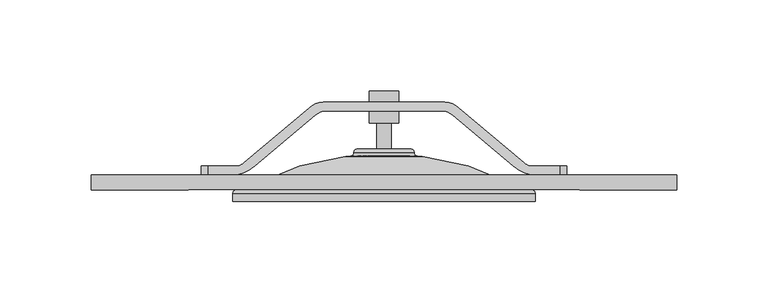
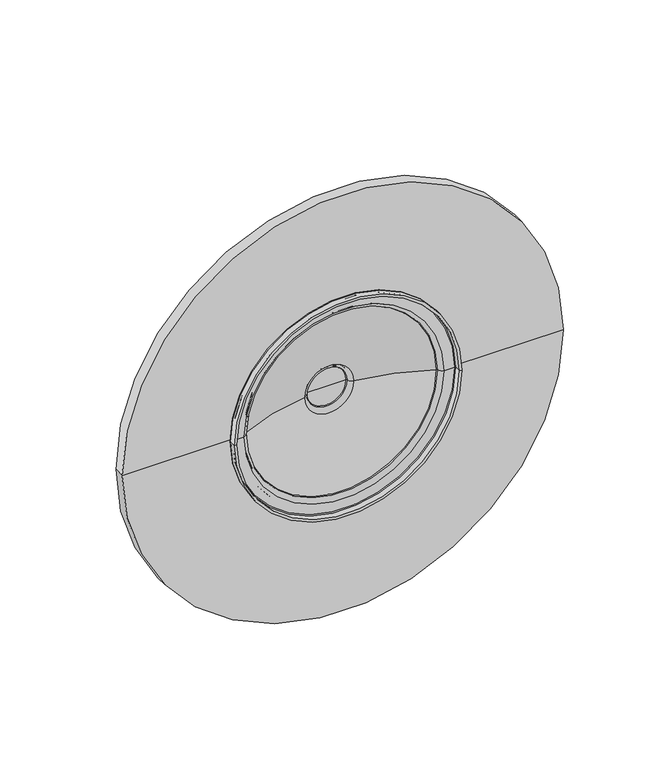
"""IFC4 building model written with IfcOpenShell, lengths in millimetres: proxy geometry, BVNC 300 8Y. : BVNC 300 8Y."""

import ifcopenshell
import ifcopenshell.guid

model = None  # the IFC model being written
_history = None  # IfcOwnerHistory: only IFC2X3 demands one
_inside = {}  # id of a spatial element -> (the spatial element, [elements in it])
_under = {}  # id of a project, library or spatial element -> (it, [spatial elements below it])
_declared = {}  # id of a project -> (the project, [libraries it declares])
_typed = {}  # id of a type object -> (the type object, [elements of that type])
_made_of = {}  # id of a material, layer set ... -> (it, [elements and type objects made of it])


def new_model(schema):
    """Start an empty IFC model of exactly this schema.

    Asked for "IFC4X3", IfcOpenShell would pick the latest addendum, in which some entities
    have other attributes; the version numbers below select the first issue.
    IFC2X3 requires an IfcOwnerHistory on every rooted entity: one is made here for all.
    """
    global model, _history
    if schema == "IFC4X3":
        model = ifcopenshell.file(schema_version=(4, 3, 0, 0))
    else:
        model = ifcopenshell.file(schema=schema)
    _inside.clear()
    _under.clear()
    _declared.clear()
    _typed.clear()
    _made_of.clear()
    _history = None
    if model.schema == "IFC2X3":
        org = make("IfcOrganization", Name="unknown")
        user = make(
            "IfcPersonAndOrganization",
            ThePerson=make("IfcPerson", FamilyName="unknown"),
            TheOrganization=org,
        )
        app = make(
            "IfcApplication",
            ApplicationDeveloper=org,
            Version="unknown",
            ApplicationFullName="unknown",
            ApplicationIdentifier="unknown",
        )
        _history = make(
            "IfcOwnerHistory",
            OwningUser=user,
            OwningApplication=app,
            ChangeAction="ADDED",
            CreationDate=0,
        )
    return model


def make(cls, **values):
    """One entity of the class cls with the attributes given. An attribute that is None is left unset."""
    return model.create_entity(
        cls, **{name: value for name, value in values.items() if value is not None}
    )


def rooted(cls, **values):
    """An entity with a GlobalId (a new one), such as an element, a storey or a relation."""
    return make(cls, GlobalId=ifcopenshell.guid.new(), OwnerHistory=_history, **values)


def si_unit(unit_type, name, prefix=None):
    """IfcSIUnit, for example si_unit("LENGTHUNIT", "METRE", prefix="MILLI")."""
    return make("IfcSIUnit", UnitType=unit_type, Prefix=prefix, Name=name)


def assignment(units):
    """IfcUnitAssignment: the units of a project."""
    return None if units is None else make("IfcUnitAssignment", Units=units)


def point(xyz):
    """IfcCartesianPoint."""
    return None if xyz is None else make("IfcCartesianPoint", Coordinates=xyz)


def direction(xyz):
    """IfcDirection."""
    return None if xyz is None else make("IfcDirection", DirectionRatios=xyz)


def frame(location, z_axis=None, x_axis=None):
    """IfcAxis2Placement3D, a coordinate frame: its origin and axes. An axis left out is left unset."""
    return make(
        "IfcAxis2Placement3D",
        Location=point(location),
        Axis=direction(z_axis),
        RefDirection=direction(x_axis),
    )


def origin():
    """The frame at (0, 0, 0) with its axes left unset."""
    return frame((0.0, 0.0, 0.0))


def place(relative_to, where):
    """IfcLocalPlacement: puts the frame where relative to a parent placement (None: the world)."""
    return make(
        "IfcLocalPlacement", PlacementRelTo=relative_to, RelativePlacement=where
    )


def context(
    kind, dimensions, precision=None, world=None, true_north=None, identifier=None
):
    """IfcGeometricRepresentationContext, for example the 3D "Model" context."""
    return make(
        "IfcGeometricRepresentationContext",
        ContextIdentifier=identifier,
        ContextType=kind,
        CoordinateSpaceDimension=dimensions,
        Precision=precision,
        WorldCoordinateSystem=world,
        TrueNorth=true_north,
    )


def project(units=None, contexts=None):
    """IfcProject with its units and contexts."""
    return rooted(
        "IfcProject",
        Name="project",
        RepresentationContexts=contexts,
        UnitsInContext=assignment(units),
    )


def spatial(cls, under=None, at=None, **own):
    """A site, building, storey or space (cls), placed at a placement, below another one or the project."""
    s = rooted(cls, ObjectPlacement=at, **own)
    if under is not None:
        _under.setdefault(under.id(), (under, []))[1].append(s)
    return s


def polyline(points):
    """IfcPolyline through the points."""
    return make("IfcPolyline", Points=[point(p) for p in points])


def circle_curve(where, radius):
    """IfcCircle in the frame where."""
    return make("IfcCircle", Position=where, Radius=radius)


def ellipse_curve(where, semi_axis1, semi_axis2):
    """IfcEllipse in the frame where."""
    return make(
        "IfcEllipse", Position=where, SemiAxis1=semi_axis1, SemiAxis2=semi_axis2
    )


def trimmed(basis, trim1, trim2, sense, master):
    """IfcTrimmedCurve: the piece of a basis curve between two trims."""
    return make(
        "IfcTrimmedCurve",
        BasisCurve=basis,
        Trim1=trim1,
        Trim2=trim2,
        SenseAgreement=sense,
        MasterRepresentation=master,
    )


def shape(context_of_items, identifier, shape_type, items):
    """IfcShapeRepresentation: the items that make up one representation, for example the "Body"."""
    return make(
        "IfcShapeRepresentation",
        ContextOfItems=context_of_items,
        RepresentationIdentifier=identifier,
        RepresentationType=shape_type,
        Items=items,
    )


def source(mapping_origin, context_of_items, identifier, shape_type, items):
    """IfcRepresentationMap: a shape defined once, which mapped items show again and again."""
    return make(
        "IfcRepresentationMap",
        MappingOrigin=mapping_origin,
        MappedRepresentation=shape(context_of_items, identifier, shape_type, items),
    )


def transform(
    local_origin,
    x_axis=None,
    y_axis=None,
    z_axis=None,
    scale=None,
    scale2=None,
    scale3=None,
    uniform=True,
):
    """IfcCartesianTransformationOperator3D, or its non-uniform kind. x_axis, y_axis, z_axis: its Axis1, 2, 3."""
    if uniform:
        return make(
            "IfcCartesianTransformationOperator3D",
            Axis1=direction(x_axis),
            Axis2=direction(y_axis),
            LocalOrigin=point(local_origin),
            Scale=scale,
            Axis3=direction(z_axis),
        )
    return make(
        "IfcCartesianTransformationOperator3DnonUniform",
        Axis1=direction(x_axis),
        Axis2=direction(y_axis),
        LocalOrigin=point(local_origin),
        Scale=scale,
        Axis3=direction(z_axis),
        Scale2=scale2,
        Scale3=scale3,
    )


def mapped(mapping_source, mapping_target):
    """IfcMappedItem: shows the shape of a source again, moved by a transform."""
    return make(
        "IfcMappedItem", MappingSource=mapping_source, MappingTarget=mapping_target
    )


def made_of(thing, what):
    """Note that an element or type object is made of a material, layer set ...; save() writes the relation."""
    if what is not None:
        _made_of.setdefault(what.id(), (what, []))[1].append(thing)
    return thing


def element(
    cls,
    number,
    at=None,
    inside=None,
    cuts=None,
    type_object=None,
    material=None,
    context=None,
    identifier="Body",
    shape_type=None,
    held_by="IfcProductDefinitionShape",
    body=None,
    shapes=None,
    **own,
):
    """One element of the class cls, such as IfcWall. Its Tag is "e" and its number.

    at: its placement. inside: the storey or other place that contains it. cuts: it is an
    opening in that element (IfcRelVoidsElement). A single representation is given by context,
    identifier, shape_type and body (its items); several are given by shapes. held_by: the class
    of the entity that holds the representations. save() writes the other relations.
    """
    e = rooted(cls, Tag="e%d" % number, ObjectPlacement=at, **own)
    if body is not None:
        shapes = [shape(context, identifier, shape_type, body)]
    if shapes is not None:
        e.Representation = make(held_by, Representations=shapes)
    if inside is not None:
        _inside.setdefault(inside.id(), (inside, []))[1].append(e)
    if cuts is not None:
        rooted(
            "IfcRelVoidsElement", RelatingBuildingElement=cuts, RelatedOpeningElement=e
        )
    if type_object is not None:
        _typed.setdefault(type_object.id(), (type_object, []))[1].append(e)
    return made_of(e, material)


def aggregate(whole, parts):
    """IfcRelAggregates: a whole, such as a stair, and the parts it consists of."""
    return rooted("IfcRelAggregates", RelatingObject=whole, RelatedObjects=parts)


def save(model, path):
    """Write the relations noted so far, then the file.

    IfcRelAggregates (storeys below a building ...), IfcRelContainedInSpatialStructure (elements
    in a storey), IfcRelDefinesByType, IfcRelAssociatesMaterial and IfcRelDeclares: one each for
    every whole, place, type object, material and project.
    """
    for whole, parts in _under.values():
        aggregate(whole, parts)
    for where, things in _inside.values():
        rooted(
            "IfcRelContainedInSpatialStructure",
            RelatedElements=things,
            RelatingStructure=where,
        )
    for kind, things in _typed.values():
        rooted("IfcRelDefinesByType", RelatedObjects=things, RelatingType=kind)
    for what, things in _made_of.values():
        rooted("IfcRelAssociatesMaterial", RelatedObjects=things, RelatingMaterial=what)
    for by, libraries in _declared.values():
        rooted("IfcRelDeclares", RelatingContext=by, RelatedDefinitions=libraries)
    model.write(path)


def plane_surface(at):
    """IfcPlane: the flat surface through the origin of the frame at, square to its z axis."""
    return make("IfcPlane", Position=at)


def cylinder_surface(at, radius):
    """IfcCylindricalSurface: all points at the distance radius from the z axis of the frame at."""
    return make("IfcCylindricalSurface", Position=at, Radius=radius)


def revolved_surface(curve, axis_point, axis_direction):
    """IfcSurfaceOfRevolution: the curve turned about the line through axis_point along axis_direction."""
    return make(
        "IfcSurfaceOfRevolution",
        SweptCurve=make("IfcArbitraryOpenProfileDef", ProfileType="CURVE", Curve=curve),
        AxisPosition=make("IfcAxis1Placement", Location=point(axis_point), Axis=direction(axis_direction)),
    )


def advanced_brep(points, edges, surfaces, faces):
    """IfcAdvancedBrep: a solid bounded by faces that lie on surfaces and meet in shared edges.

    An edge is (start, end): straight between two places in points (the first is 0);
    or (start, end, curve); or (start, end, curve, False) where it runs against its curve.
    A face is (place in surfaces, loops), or (place, loops, False) where it looks against
    its surface's normal. A loop lists edges by number (the first is 1), with a minus sign
    where the edge is run from its end to its start. The first loop is the outer one.
    """
    corners = [point(p) for p in points]
    vertices = [make("IfcVertexPoint", VertexGeometry=c) for c in corners]
    made = []
    for start, end, *more in edges:
        made.append(
            make(
                "IfcEdgeCurve",
                EdgeStart=vertices[start],
                EdgeEnd=vertices[end],
                EdgeGeometry=more[0] if more else make("IfcPolyline", Points=[corners[start], corners[end]]),
                SameSense=more[1] if len(more) > 1 else True,
            )
        )
    hull = []
    for where, loops, *sense in faces:
        bounds = []
        for j, loop in enumerate(loops):
            ring = [make("IfcOrientedEdge", EdgeElement=made[abs(k) - 1], Orientation=k > 0) for k in loop]
            bounds.append(
                make(
                    "IfcFaceOuterBound" if j == 0 else "IfcFaceBound",
                    Bound=make("IfcEdgeLoop", EdgeList=ring),
                    Orientation=True,
                )
            )
        hull.append(make("IfcAdvancedFace", Bounds=bounds, FaceSurface=surfaces[where], SameSense=sense[0] if sense else True))
    return make("IfcAdvancedBrep", Outer=make("IfcClosedShell", CfsFaces=hull))


def mechanical_equipment_0198ac86(model_context):
    return source(origin(), model_context, "Body", "AdvancedBrep", [
        advanced_brep(
        [(44.3795006, 108.0, 2510.0), (54.2298211, 113.0, 2510.0), (87.44309, 140.8692417, 2510.0), (91.8102497, 143.0, 2510.0), (125.0, 143.0, 2510.0), (158.1897503, 143.0, 2510.0), (162.55691, 140.8692417, 2510.0), (195.7701789, 113.0, 2510.0), (205.6204994, 108.0, 2510.0), (221.2200072, 108.0, 2510.0), (221.2200072, 113.0, 2510.0), (205.6204994, 113.0, 2510.0), (201.5540671, 114.8851429, 2510.0), (165.874925, 144.8234979, 2510.0), (158.1897503, 148.0, 2510.0), (125.0, 148.0, 2510.0), (91.8102497, 148.0, 2510.0), (84.125075, 144.8234979, 2510.0), (48.4459329, 114.8851429, 2510.0), (44.3795006, 113.0, 2510.0), (28.7799928, 113.0, 2510.0), (28.7799928, 108.0, 2510.0), (44.3795006, 113.0, 2490.0), (48.4459329, 114.8851429, 2490.0), (84.125075, 144.8234979, 2490.0), (91.8102497, 148.0, 2490.0), (125.0, 148.0, 2490.0), (158.1897503, 148.0, 2490.0), (165.874925, 144.8234979, 2490.0), (201.5540671, 114.8851429, 2490.0), (205.6204994, 113.0, 2490.0), (221.2200072, 113.0, 2490.0), (221.2200072, 108.0, 2490.0), (205.6204994, 108.0, 2490.0), (195.7701789, 113.0, 2490.0), (162.55691, 140.8692417, 2490.0), (158.1897503, 143.0, 2490.0), (125.0, 143.0, 2490.0), (91.8102497, 143.0, 2490.0), (87.44309, 140.8692417, 2490.0), (54.2298211, 113.0, 2490.0), (44.3795006, 108.0, 2490.0), (28.7799928, 108.0, 2490.0), (28.7799928, 113.0, 2490.0), (25.0, 108.0, 2506.2200072), (25.0, 108.0, 2493.7799928), (225.0, 108.0, 2493.7799928), (225.0, 108.0, 2506.2200072), (225.0, 113.0, 2493.7799928), (225.0, 113.0, 2506.2200072), (25.0, 113.0, 2493.7799928), (25.0, 113.0, 2506.2200072)],
        [
            (0, 1, circle_curve(frame((38.5511411, 131.6851233, 2510.0), z_axis=(0.0, 0.0, 1.0), x_axis=(1.0, 0.0, 0.0)), 24.3916961)),
            (1, 2),
            (2, 3, circle_curve(frame((93.9022065, 133.1715663, 2510.0), z_axis=(0.0, 0.0, -1.0), x_axis=(1.0, 0.0, 0.0)), 10.0486015)),
            (3, 4),
            (4, 5),
            (5, 6, circle_curve(frame((156.0977935, 133.1715663, 2510.0), z_axis=(0.0, 0.0, -1.0), x_axis=(-1.0, 0.0, 0.0)), 10.0486015)),
            (6, 7),
            (7, 8, circle_curve(frame((211.4488589, 131.6851233, 2510.0), z_axis=(0.0, 0.0, 1.0), x_axis=(-1.0, 0.0, 0.0)), 24.3916961)),
            (8, 9),
            (9, 10),
            (10, 11),
            (11, 12, circle_curve(frame((205.6204994, 118.3284116, 2510.0), z_axis=(0.0, 0.0, -1.0), x_axis=(-1.0, 0.0, 0.0)), 5.3284116)),
            (12, 13),
            (13, 14, circle_curve(frame((158.1897503, 137.115059, 2510.0), z_axis=(0.0, 0.0, 1.0), x_axis=(-1.0, 0.0, 0.0)), 10.884941)),
            (14, 15),
            (15, 16),
            (16, 17, circle_curve(frame((91.8102497, 137.115059, 2510.0), z_axis=(0.0, 0.0, 1.0), x_axis=(1.0, 0.0, 0.0)), 10.884941)),
            (17, 18),
            (18, 19, circle_curve(frame((44.3795006, 118.3284116, 2510.0), z_axis=(0.0, 0.0, -1.0), x_axis=(1.0, 0.0, 0.0)), 5.3284116)),
            (19, 20),
            (20, 21),
            (21, 0),
            (22, 23, circle_curve(frame((44.3795006, 118.3284116, 2490.0), z_axis=(0.0, 0.0, 1.0), x_axis=(1.0, 0.0, 0.0)), 5.3284116)),
            (23, 24),
            (24, 25, circle_curve(frame((91.8102497, 137.115059, 2490.0), z_axis=(0.0, 0.0, -1.0), x_axis=(1.0, 0.0, 0.0)), 10.884941)),
            (25, 26),
            (26, 27),
            (27, 28, circle_curve(frame((158.1897503, 137.115059, 2490.0), z_axis=(0.0, 0.0, -1.0), x_axis=(-1.0, 0.0, 0.0)), 10.884941)),
            (28, 29),
            (29, 30, circle_curve(frame((205.6204994, 118.3284116, 2490.0), z_axis=(0.0, 0.0, 1.0), x_axis=(-1.0, 0.0, 0.0)), 5.3284116)),
            (30, 31),
            (31, 32),
            (32, 33),
            (33, 34, circle_curve(frame((211.4488589, 131.6851233, 2490.0), z_axis=(0.0, 0.0, -1.0), x_axis=(-1.0, 0.0, 0.0)), 24.3916961)),
            (34, 35),
            (35, 36, circle_curve(frame((156.0977935, 133.1715663, 2490.0), z_axis=(0.0, 0.0, 1.0), x_axis=(-1.0, 0.0, 0.0)), 10.0486015)),
            (36, 37),
            (37, 38),
            (38, 39, circle_curve(frame((93.9022065, 133.1715663, 2490.0), z_axis=(0.0, 0.0, 1.0), x_axis=(1.0, 0.0, 0.0)), 10.0486015)),
            (39, 40),
            (40, 41, circle_curve(frame((38.5511411, 131.6851233, 2490.0), z_axis=(0.0, 0.0, -1.0), x_axis=(1.0, 0.0, 0.0)), 24.3916961)),
            (41, 42),
            (42, 43),
            (43, 22),
            (41, 0),
            (21, 44, circle_curve(frame((28.7799928, 108.0, 2506.2200072), z_axis=(0.0, -1.0, 0.0), x_axis=(1.0, 0.0, 0.0)), 3.7799928)),
            (44, 45),
            (45, 42, circle_curve(frame((28.7799928, 108.0, 2493.7799928), z_axis=(0.0, -1.0, 0.0), x_axis=(1.0, 0.0, 0.0)), 3.7799928)),
            (40, 1),
            (39, 2),
            (38, 3),
            (37, 4),
            (36, 5),
            (35, 6),
            (34, 7),
            (33, 8),
            (32, 46, circle_curve(frame((221.2200072, 108.0, 2493.7799928), z_axis=(0.0, -1.0, 0.0), x_axis=(-1.0, 0.0, 0.0)), 3.7799928)),
            (46, 47),
            (47, 9, circle_curve(frame((221.2200072, 108.0, 2506.2200072), z_axis=(0.0, -1.0, 0.0), x_axis=(-1.0, 0.0, 0.0)), 3.7799928)),
            (46, 48),
            (48, 49),
            (49, 47),
            (30, 11),
            (10, 49, circle_curve(frame((221.2200072, 113.0, 2506.2200072), z_axis=(0.0, 1.0, 0.0), x_axis=(-1.0, 0.0, 0.0)), 3.7799928)),
            (48, 31, circle_curve(frame((221.2200072, 113.0, 2493.7799928), z_axis=(0.0, 1.0, 0.0), x_axis=(-1.0, 0.0, 0.0)), 3.7799928)),
            (29, 12),
            (28, 13),
            (27, 14),
            (26, 15),
            (25, 16),
            (24, 17),
            (23, 18),
            (22, 19),
            (43, 50, circle_curve(frame((28.7799928, 113.0, 2493.7799928), z_axis=(0.0, 1.0, 0.0), x_axis=(1.0, 0.0, 0.0)), 3.7799928)),
            (50, 51),
            (51, 20, circle_curve(frame((28.7799928, 113.0, 2506.2200072), z_axis=(0.0, 1.0, 0.0), x_axis=(1.0, 0.0, 0.0)), 3.7799928)),
            (44, 51),
            (50, 45),
        ],
        [
            plane_surface(frame((25.0, 108.0, 2510.0), z_axis=(0.0, 0.0, 1.0), x_axis=(1.0, 0.0, 0.0))),
            plane_surface(frame((25.0, 108.0, 2490.0), z_axis=(0.0, 0.0, -1.0), x_axis=(-1.0, 0.0, 0.0))),
            plane_surface(frame((25.0, 108.0, 2510.0), z_axis=(0.0, -1.0, 0.0), x_axis=(0.0, 0.0, -1.0))),
            cylinder_surface(frame((38.5511411, 131.6851233, 2490.0), z_axis=(0.0, 0.0, 1.0), x_axis=(1.0, 0.0, 0.0)), 24.3916961),
            plane_surface(frame((54.2298211, 113.0, 2510.0), z_axis=(0.6427876096865391, -0.7660444431189783, 0.0), x_axis=(0.0, 0.0, -1.0))),
            revolved_surface(polyline([(103.95080800000001, 133.1715663, 2490.0), (103.95080800000001, 133.1715663, 2510.0)]), (93.9022065, 133.1715663, 2490.0), (0.0, 0.0, -1.0)),
            plane_surface(frame((91.8102497, 143.0, 2510.0), z_axis=(0.0, -1.0, 0.0), x_axis=(0.0, 0.0, -1.0))),
            plane_surface(frame((125.0, 143.0, 2510.0), z_axis=(0.0, -1.0, 0.0), x_axis=(0.0, 0.0, -1.0))),
            revolved_surface(polyline([(146.049192, 133.1715663, 2490.0), (146.049192, 133.1715663, 2510.0)]), (156.0977935, 133.1715663, 2490.0), (0.0, 0.0, -1.0)),
            plane_surface(frame((162.55691, 140.8692417, 2510.0), z_axis=(-0.6427876096865387, -0.7660444431189786, 0.0), x_axis=(0.0, 0.0, -1.0))),
            cylinder_surface(frame((211.4488589, 131.6851233, 2490.0), z_axis=(0.0, 0.0, 1.0), x_axis=(-1.0, 0.0, 0.0)), 24.3916961),
            plane_surface(frame((205.6204994, 108.0, 2510.0), z_axis=(0.0, -1.0, 0.0), x_axis=(0.0, 0.0, -1.0))),
            plane_surface(frame((225.0, 108.0, 2510.0), z_axis=(1.0, 0.0, 0.0), x_axis=(0.0, 0.0, -1.0))),
            plane_surface(frame((225.0, 113.0, 2510.0), z_axis=(0.0, 1.0, 0.0), x_axis=(0.0, 0.0, -1.0))),
            revolved_surface(polyline([(200.2920878, 118.3284116, 2490.0), (200.2920878, 118.3284116, 2510.0)]), (205.6204994, 118.3284116, 2490.0), (0.0, 0.0, -1.0)),
            plane_surface(frame((201.5540671, 114.8851429, 2510.0), z_axis=(0.6427876096865414, 0.7660444431189763, 0.0), x_axis=(0.0, 0.0, -1.0))),
            cylinder_surface(frame((158.1897503, 137.115059, 2490.0), z_axis=(0.0, 0.0, 1.0), x_axis=(-1.0, 0.0, 0.0)), 10.884941),
            plane_surface(frame((158.1897503, 148.0, 2510.0), z_axis=(0.0, 1.0, 0.0), x_axis=(0.0, 0.0, -1.0))),
            plane_surface(frame((125.0, 148.0, 2510.0), z_axis=(0.0, 1.0, 0.0), x_axis=(0.0, 0.0, -1.0))),
            cylinder_surface(frame((91.8102497, 137.115059, 2490.0), z_axis=(0.0, 0.0, 1.0), x_axis=(1.0, 0.0, 0.0)), 10.884941),
            plane_surface(frame((84.125075, 144.8234979, 2510.0), z_axis=(-0.6427876096865359, 0.766044443118981, 0.0), x_axis=(0.0, 0.0, -1.0))),
            revolved_surface(polyline([(49.7079122, 118.3284116, 2490.0), (49.7079122, 118.3284116, 2510.0)]), (44.3795006, 118.3284116, 2490.0), (0.0, 0.0, -1.0)),
            plane_surface(frame((44.3795006, 113.0, 2510.0), z_axis=(0.0, 1.0, 0.0), x_axis=(0.0, 0.0, -1.0))),
            plane_surface(frame((25.0, 113.0, 2510.0), z_axis=(-1.0, 0.0, 0.0), x_axis=(0.0, 0.0, -1.0))),
            cylinder_surface(frame((28.7799928, 108.0, 2493.7799928), z_axis=(0.0, -1.0, 0.0), x_axis=(1.0, 0.0, 0.0)), 3.7799928),
            cylinder_surface(frame((28.7799928, 93.5, 2506.2200072), z_axis=(0.0, -1.0, 0.0), x_axis=(1.0, 0.0, 0.0)), 3.7799928),
            cylinder_surface(frame((221.2200072, 93.5, 2493.7799928), z_axis=(0.0, -1.0, 0.0), x_axis=(-1.0, 0.0, 0.0)), 3.7799928),
            cylinder_surface(frame((221.2200072, 93.5, 2506.2200072), z_axis=(0.0, -1.0, 0.0), x_axis=(-1.0, 0.0, 0.0)), 3.7799928),
        ],
        [
            (0, [[1, 2, 3, 4, 5, 6, 7, 8, 9, 10, 11, 12, 13, 14, 15, 16, 17, 18, 19, 20, 21, 22]]),
            (1, [[23, 24, 25, 26, 27, 28, 29, 30, 31, 32, 33, 34, 35, 36, 37, 38, 39, 40, 41, 42, 43, 44]]),
            (2, [[45, -22, 46, 47, 48, -42]]),
            (3, [[-1, -45, -41, 49]]),
            (4, [[-2, -49, -40, 50]]),
            (5, [[-3, -50, -39, 51]]),
            (6, [[-4, -51, -38, 52]]),
            (7, [[-5, -52, -37, 53]]),
            (8, [[-6, -53, -36, 54]]),
            (9, [[-7, -54, -35, 55]]),
            (10, [[-8, -55, -34, 56]]),
            (11, [[-56, -33, 57, 58, 59, -9]]),
            (12, [[-58, 60, 61, 62]]),
            (13, [[63, -11, 64, -61, 65, -31]]),
            (14, [[-12, -63, -30, 66]]),
            (15, [[-13, -66, -29, 67]]),
            (16, [[-14, -67, -28, 68]]),
            (17, [[-15, -68, -27, 69]]),
            (18, [[-16, -69, -26, 70]]),
            (19, [[-17, -70, -25, 71]]),
            (20, [[-18, -71, -24, 72]]),
            (21, [[-19, -72, -23, 73]]),
            (22, [[-73, -44, 74, 75, 76, -20]]),
            (23, [[-47, 77, -75, 78]]),
            (24, [[-43, -48, -78, -74]]),
            (25, [[-21, -76, -77, -46]]),
            (26, [[-32, -65, -60, -57]]),
            (27, [[-10, -59, -62, -64]]),
        ],
    ),
        advanced_brep(
        [(207.7271571, 93.5, 2500.0), (42.2728429, 93.5, 2500.0), (42.2728429, 97.7728429, 2500.0), (207.7271571, 97.7728429, 2500.0), (205.9367462, 93.5, 2500.0), (44.0632538, 93.5, 2500.0), (205.9367462, 97.9071057, 2500.0), (44.0632538, 97.9071057, 2500.0), (205.3438519, 98.5, 2500.0), (44.6561481, 98.5, 2500.0), (197.7785514, 98.5, 2500.0), (52.2214486, 98.5, 2500.0), (194.5390342, 101.1233093, 2500.0), (55.4609658, 101.1233093, 2500.0), (194.110594, 101.9290881, 2500.0), (55.889406, 101.9290881, 2500.0), (143.1174907, 117.056758, 2500.0), (106.8825093, 117.056758, 2500.0), (139.9690463, 120.2052024, 2500.0), (110.0309537, 120.2052024, 2500.0), (139.3942487, 120.78, 2500.0), (110.6057513, 120.78, 2500.0), (125.0, 120.78, 2500.0), (139.6388233, 122.2731901, 2500.0), (110.3611767, 122.2731901, 2500.0), (120.9566338, 122.2731901, 2500.0), (129.0433662, 122.2731901, 2500.0), (141.5029828, 120.4090307, 2500.0), (108.4970172, 120.4090307, 2500.0), (143.1991524, 118.522856, 2500.0), (106.8008476, 118.522856, 2500.0), (145.9642188, 118.2410596, 2500.0), (104.0357812, 118.2410596, 2500.0), (194.877574, 103.206216, 2500.0), (55.122426, 103.206216, 2500.0), (196.1038029, 101.6367146, 2500.0), (53.8961971, 101.6367146, 2500.0), (198.0543634, 100.0, 2500.0), (51.9456366, 100.0, 2500.0), (200.0, 100.0, 2500.0), (50.0, 100.0, 2500.0), (200.0, 108.0, 2500.0), (50.0, 108.0, 2500.0), (285.0, 108.0, 2500.0), (-35.0, 108.0, 2500.0), (285.0, 100.0, 2500.0), (-35.0, 100.0, 2500.0), (205.5, 100.0, 2500.0), (44.5, 100.0, 2500.0), (133.0867323, 136.6576943, 2500.0), (116.9132677, 136.6576943, 2500.0), (116.9132677, 153.9, 2500.0), (133.0867323, 153.9, 2500.0), (129.0433662, 136.6576943, 2500.0), (120.9566338, 136.6576943, 2500.0), (125.0, 153.9, 2500.0)],
        [
            (0, 1, circle_curve(frame((125.0, 93.5, 2500.0), z_axis=(0.0, 1.0, 0.0), x_axis=(-1.0, 0.0, 0.0)), 82.7271571)),
            (1, 2),
            (2, 3, circle_curve(frame((125.0, 97.7728429, 2500.0), z_axis=(0.0, -1.0, 0.0), x_axis=(-1.0, 0.0, 0.0)), 82.7271571)),
            (3, 0),
            (1, 0, circle_curve(frame((125.0, 93.5, 2500.0), z_axis=(0.0, 1.0, 0.0), x_axis=(-1.0, 0.0, 0.0)), 82.7271571)),
            (3, 2, circle_curve(frame((125.0, 97.7728429, 2500.0), z_axis=(0.0, -1.0, 0.0), x_axis=(-1.0, 0.0, 0.0)), 82.7271571)),
            (0, 4),
            (4, 5, circle_curve(frame((125.0, 93.5, 2500.0), z_axis=(0.0, 1.0, 0.0), x_axis=(-1.0, 0.0, 0.0)), 80.9367462)),
            (5, 1),
            (5, 4, circle_curve(frame((125.0, 93.5, 2500.0), z_axis=(0.0, 1.0, 0.0), x_axis=(-1.0, 0.0, 0.0)), 80.9367462)),
            (4, 6),
            (6, 7, circle_curve(frame((125.0, 97.9071057, 2500.0), z_axis=(0.0, 1.0, 0.0), x_axis=(-1.0, 0.0, 0.0)), 80.9367462)),
            (7, 5),
            (7, 6, circle_curve(frame((125.0, 97.9071057, 2500.0), z_axis=(0.0, 1.0, 0.0), x_axis=(-1.0, 0.0, 0.0)), 80.9367462)),
            (6, 8, circle_curve(frame((205.3438519, 97.9071057, 2500.0), z_axis=(0.0, 0.0, 1.0), x_axis=(-1.0, 0.0, 0.0)), 0.5928943)),
            (8, 9, circle_curve(frame((125.0, 98.5, 2500.0), z_axis=(0.0, 1.0, 0.0), x_axis=(-1.0, 0.0, 0.0)), 80.3438519)),
            (9, 7, circle_curve(frame((44.6561481, 97.9071057, 2500.0), z_axis=(0.0, 0.0, 1.0), x_axis=(1.0, 0.0, 0.0)), 0.5928943)),
            (9, 8, circle_curve(frame((125.0, 98.5, 2500.0), z_axis=(0.0, 1.0, 0.0), x_axis=(-1.0, 0.0, 0.0)), 80.3438519)),
            (8, 10),
            (10, 11, circle_curve(frame((125.0, 98.5, 2500.0), z_axis=(0.0, 1.0, 0.0), x_axis=(-1.0, 0.0, 0.0)), 72.7785514)),
            (11, 9),
            (11, 10, circle_curve(frame((125.0, 98.5, 2500.0), z_axis=(0.0, 1.0, 0.0), x_axis=(-1.0, 0.0, 0.0)), 72.7785514)),
            (10, 12, circle_curve(frame((197.9467336, 102.0195777, 2500.0), z_axis=(0.0, 0.0, -1.0), x_axis=(-1.0, 0.0, 0.0)), 3.5235937)),
            (12, 13, circle_curve(frame((125.0, 101.1233093, 2500.0), z_axis=(0.0, 1.0, 0.0), x_axis=(-1.0, 0.0, 0.0)), 69.5390342)),
            (13, 11, circle_curve(frame((52.0532664, 102.0195777, 2500.0), z_axis=(0.0, 0.0, -1.0), x_axis=(1.0, 0.0, 0.0)), 3.5235937)),
            (13, 12, circle_curve(frame((125.0, 101.1233093, 2500.0), z_axis=(0.0, 1.0, 0.0), x_axis=(-1.0, 0.0, 0.0)), 69.5390342)),
            (12, 14, circle_curve(frame((193.7458269, 101.2183458, 2500.0), z_axis=(0.0, 0.0, 1.0), x_axis=(-1.0, 0.0, 0.0)), 0.7988803)),
            (14, 15, circle_curve(frame((125.0, 101.9290881, 2500.0), z_axis=(0.0, 1.0, 0.0), x_axis=(-1.0, 0.0, 0.0)), 69.110594)),
            (15, 13, circle_curve(frame((56.2541731, 101.2183458, 2500.0), z_axis=(0.0, 0.0, 1.0), x_axis=(1.0, 0.0, 0.0)), 0.7988803)),
            (15, 14, circle_curve(frame((125.0, 101.9290881, 2500.0), z_axis=(0.0, 1.0, 0.0), x_axis=(-1.0, 0.0, 0.0)), 69.110594)),
            (14, 16, circle_curve(frame((128.3688639, -26.1675298, 2500.0), z_axis=(0.0, 0.0, 1.0), x_axis=(-1.0, 0.0, 0.0)), 143.9816606)),
            (16, 17, circle_curve(frame((125.0, 117.056758, 2500.0), z_axis=(0.0, 1.0, 0.0), x_axis=(-1.0, 0.0, 0.0)), 18.1174907)),
            (17, 15, circle_curve(frame((121.6311361, -26.1675298, 2500.0), z_axis=(0.0, 0.0, 1.0), x_axis=(1.0, 0.0, 0.0)), 143.9816606)),
            (17, 16, circle_curve(frame((125.0, 117.056758, 2500.0), z_axis=(0.0, 1.0, 0.0), x_axis=(-1.0, 0.0, 0.0)), 18.1174907)),
            (16, 18, circle_curve(frame((143.1174907, 120.2052024, 2500.0), z_axis=(0.0, 0.0, -1.0), x_axis=(-1.0, 0.0, 0.0)), 3.1484444)),
            (18, 19, circle_curve(frame((125.0, 120.2052024, 2500.0), z_axis=(0.0, 1.0, 0.0), x_axis=(-1.0, 0.0, 0.0)), 14.9690463)),
            (19, 17, circle_curve(frame((106.8825093, 120.2052024, 2500.0), z_axis=(0.0, 0.0, -1.0), x_axis=(1.0, 0.0, 0.0)), 3.1484444)),
            (19, 18, circle_curve(frame((125.0, 120.2052024, 2500.0), z_axis=(0.0, 1.0, 0.0), x_axis=(-1.0, 0.0, 0.0)), 14.9690463)),
            (18, 20, circle_curve(frame((139.3942487, 120.2052024, 2500.0), z_axis=(0.0, 0.0, 1.0), x_axis=(-1.0, 0.0, 0.0)), 0.5747976)),
            (20, 21, circle_curve(frame((125.0, 120.78, 2500.0), z_axis=(0.0, 1.0, 0.0), x_axis=(-1.0, 0.0, 0.0)), 14.3942487)),
            (21, 19, circle_curve(frame((110.6057513, 120.2052024, 2500.0), z_axis=(0.0, 0.0, 1.0), x_axis=(1.0, 0.0, 0.0)), 0.5747976)),
            (21, 20, circle_curve(frame((125.0, 120.78, 2500.0), z_axis=(0.0, 1.0, 0.0), x_axis=(-1.0, 0.0, 0.0)), 14.3942487)),
            (20, 22),
            (22, 21),
            (23, 24, circle_curve(frame((125.0, 122.2731901, 2500.0), z_axis=(0.0, 1.0, 0.0), x_axis=(-1.0, 0.0, 0.0)), 14.6388233)),
            (24, 25),
            (25, 26, circle_curve(frame((125.0, 122.2731901, 2500.0), z_axis=(0.0, -1.0, 0.0), x_axis=(-1.0, 0.0, 0.0)), 4.0433662)),
            (26, 23),
            (24, 23, circle_curve(frame((125.0, 122.2731901, 2500.0), z_axis=(0.0, 1.0, 0.0), x_axis=(-1.0, 0.0, 0.0)), 14.6388233)),
            (26, 25, circle_curve(frame((125.0, 122.2731901, 2500.0), z_axis=(0.0, -1.0, 0.0), x_axis=(-1.0, 0.0, 0.0)), 4.0433662)),
            (23, 27, circle_curve(frame((139.6388233, 120.4090307, 2500.0), z_axis=(0.0, 0.0, -1.0), x_axis=(-1.0, 0.0, 0.0)), 1.8641595)),
            (27, 28, circle_curve(frame((125.0, 120.4090307, 2500.0), z_axis=(0.0, 1.0, 0.0), x_axis=(-1.0, 0.0, 0.0)), 16.5029828)),
            (28, 24, circle_curve(frame((110.3611767, 120.4090307, 2500.0), z_axis=(0.0, 0.0, -1.0), x_axis=(1.0, 0.0, 0.0)), 1.8641595)),
            (28, 27, circle_curve(frame((125.0, 120.4090307, 2500.0), z_axis=(0.0, 1.0, 0.0), x_axis=(-1.0, 0.0, 0.0)), 16.5029828)),
            (27, 29, circle_curve(frame((143.3997997, 120.4090307, 2500.0), z_axis=(0.0, 0.0, 1.0), x_axis=(-1.0, 0.0, 0.0)), 1.8968169)),
            (29, 30, circle_curve(frame((125.0, 118.522856, 2500.0), z_axis=(0.0, 1.0, 0.0), x_axis=(-1.0, 0.0, 0.0)), 18.1991524)),
            (30, 28, circle_curve(frame((106.6002003, 120.4090307, 2500.0), z_axis=(0.0, 0.0, 1.0), x_axis=(1.0, 0.0, 0.0)), 1.8968169)),
            (30, 29, circle_curve(frame((125.0, 118.522856, 2500.0), z_axis=(0.0, 1.0, 0.0), x_axis=(-1.0, 0.0, 0.0)), 18.1991524)),
            (29, 31, circle_curve(frame((176.4809645, 431.386753, 2500.0), z_axis=(0.0, 0.0, 1.0), x_axis=(-1.0, 0.0, 0.0)), 314.6291421)),
            (31, 32, circle_curve(frame((125.0, 118.2410596, 2500.0), z_axis=(0.0, 1.0, 0.0), x_axis=(-1.0, 0.0, 0.0)), 20.9642188)),
            (32, 30, circle_curve(frame((73.5190355, 431.386753, 2500.0), z_axis=(0.0, 0.0, 1.0), x_axis=(1.0, 0.0, 0.0)), 314.6291421)),
            (32, 31, circle_curve(frame((125.0, 118.2410596, 2500.0), z_axis=(0.0, 1.0, 0.0), x_axis=(-1.0, 0.0, 0.0)), 20.9642188)),
            (31, 33, circle_curve(frame((131.9555378, -14.4169888, 2500.0), z_axis=(0.0, 0.0, -1.0), x_axis=(-1.0, 0.0, 0.0)), 133.3956557)),
            (33, 34, circle_curve(frame((125.0, 103.206216, 2500.0), z_axis=(0.0, 1.0, 0.0), x_axis=(-1.0, 0.0, 0.0)), 69.877574)),
            (34, 32, circle_curve(frame((118.0444622, -14.4169888, 2500.0), z_axis=(0.0, 0.0, -1.0), x_axis=(1.0, 0.0, 0.0)), 133.3956557)),
            (34, 33, circle_curve(frame((125.0, 103.206216, 2500.0), z_axis=(0.0, 1.0, 0.0), x_axis=(-1.0, 0.0, 0.0)), 69.877574)),
            (33, 35, circle_curve(frame((194.0147871, 101.2683648, 2500.0), z_axis=(0.0, 0.0, -1.0), x_axis=(-1.0, 0.0, 0.0)), 2.1212422)),
            (35, 36, circle_curve(frame((125.0, 101.6367146, 2500.0), z_axis=(0.0, 1.0, 0.0), x_axis=(-1.0, 0.0, 0.0)), 71.1038029)),
            (36, 34, circle_curve(frame((55.9852129, 101.2683648, 2500.0), z_axis=(0.0, 0.0, -1.0), x_axis=(1.0, 0.0, 0.0)), 2.1212422)),
            (36, 35, circle_curve(frame((125.0, 101.6367146, 2500.0), z_axis=(0.0, 1.0, 0.0), x_axis=(-1.0, 0.0, 0.0)), 71.1038029)),
            (35, 37, circle_curve(frame((198.0543634, 101.9806511, 2500.0), z_axis=(0.0, 0.0, 1.0), x_axis=(-1.0, 0.0, 0.0)), 1.9806511)),
            (37, 38, circle_curve(frame((125.0, 100.0, 2500.0), z_axis=(0.0, 1.0, 0.0), x_axis=(-1.0, 0.0, 0.0)), 73.0543634)),
            (38, 36, circle_curve(frame((51.9456366, 101.9806511, 2500.0), z_axis=(0.0, 0.0, 1.0), x_axis=(1.0, 0.0, 0.0)), 1.9806511)),
            (38, 37, circle_curve(frame((125.0, 100.0, 2500.0), z_axis=(0.0, 1.0, 0.0), x_axis=(-1.0, 0.0, 0.0)), 73.0543634)),
            (37, 39),
            (39, 40, circle_curve(frame((125.0, 100.0, 2500.0), z_axis=(0.0, 1.0, 0.0), x_axis=(-1.0, 0.0, 0.0)), 75.0)),
            (40, 38),
            (40, 39, circle_curve(frame((125.0, 100.0, 2500.0), z_axis=(0.0, 1.0, 0.0), x_axis=(-1.0, 0.0, 0.0)), 75.0)),
            (39, 41),
            (41, 42, circle_curve(frame((125.0, 108.0, 2500.0), z_axis=(0.0, 1.0, 0.0), x_axis=(-1.0, 0.0, 0.0)), 75.0)),
            (42, 40),
            (42, 41, circle_curve(frame((125.0, 108.0, 2500.0), z_axis=(0.0, 1.0, 0.0), x_axis=(-1.0, 0.0, 0.0)), 75.0)),
            (41, 43),
            (43, 44, circle_curve(frame((125.0, 108.0, 2500.0), z_axis=(0.0, 1.0, 0.0), x_axis=(-1.0, 0.0, 0.0)), 160.0)),
            (44, 42),
            (44, 43, circle_curve(frame((125.0, 108.0, 2500.0), z_axis=(0.0, 1.0, 0.0), x_axis=(-1.0, 0.0, 0.0)), 160.0)),
            (43, 45),
            (45, 46, circle_curve(frame((125.0, 100.0, 2500.0), z_axis=(0.0, 1.0, 0.0), x_axis=(-1.0, 0.0, 0.0)), 160.0)),
            (46, 44),
            (46, 45, circle_curve(frame((125.0, 100.0, 2500.0), z_axis=(0.0, 1.0, 0.0), x_axis=(-1.0, 0.0, 0.0)), 160.0)),
            (45, 47),
            (47, 48, circle_curve(frame((125.0, 100.0, 2500.0), z_axis=(0.0, 1.0, 0.0), x_axis=(-1.0, 0.0, 0.0)), 80.5)),
            (48, 46),
            (48, 47, circle_curve(frame((125.0, 100.0, 2500.0), z_axis=(0.0, 1.0, 0.0), x_axis=(-1.0, 0.0, 0.0)), 80.5)),
            (2, 48, circle_curve(frame((44.5, 97.7728429, 2500.0), z_axis=(0.0, 0.0, -1.0), x_axis=(1.0, 0.0, 0.0)), 2.2271571)),
            (47, 3, circle_curve(frame((205.5, 97.7728429, 2500.0), z_axis=(0.0, 0.0, -1.0), x_axis=(-1.0, 0.0, 0.0)), 2.2271571)),
            (49, 50, circle_curve(frame((125.0, 136.6576943, 2500.0), z_axis=(0.0, 1.0, 0.0), x_axis=(-1.0, 0.0, 0.0)), 8.0867323)),
            (50, 51),
            (51, 52, circle_curve(frame((125.0, 153.9, 2500.0), z_axis=(0.0, -1.0, 0.0), x_axis=(-1.0, 0.0, 0.0)), 8.0867323)),
            (52, 49),
            (50, 49, circle_curve(frame((125.0, 136.6576943, 2500.0), z_axis=(0.0, 1.0, 0.0), x_axis=(-1.0, 0.0, 0.0)), 8.0867323)),
            (52, 51, circle_curve(frame((125.0, 153.9, 2500.0), z_axis=(0.0, -1.0, 0.0), x_axis=(-1.0, 0.0, 0.0)), 8.0867323)),
            (49, 53),
            (53, 54, circle_curve(frame((125.0, 136.6576943, 2500.0), z_axis=(0.0, 1.0, 0.0), x_axis=(-1.0, 0.0, 0.0)), 4.0433662)),
            (54, 50),
            (54, 53, circle_curve(frame((125.0, 136.6576943, 2500.0), z_axis=(0.0, 1.0, 0.0), x_axis=(-1.0, 0.0, 0.0)), 4.0433662)),
            (51, 55),
            (55, 52),
            (25, 54),
            (53, 26),
        ],
        [
            cylinder_surface(frame((125.0, 193.5, 2500.0), z_axis=(0.0, -1.0, 0.0), x_axis=(-1.0, 0.0, 0.0)), 82.7271571),
            plane_surface(frame((125.0, 93.5, 2500.0), z_axis=(0.0, -1.0, 0.0), x_axis=(-1.0, 0.0, 0.0))),
            revolved_surface(polyline([(44.0632538, 93.5, 2500.0), (44.0632538, 97.9071057, 2500.0)]), (125.0, 193.5, 2500.0), (0.0, -1.0, 0.0)),
            revolved_surface(trimmed(ellipse_curve(frame((44.6561481, 97.9071057, 2500.0), z_axis=(0.0, 0.0, -1.0), x_axis=(1.0, 0.0, 0.0)), 0.5928943, 0.5928943), [point((44.0632538, 97.9071057, 2500.0))], [point((44.6561481, 98.5, 2500.0))], True, "CARTESIAN"), (125.0, 193.5, 2500.0), (0.0, -1.0, 0.0)),
            plane_surface(frame((125.0, 98.5, 2500.0), z_axis=(0.0, -1.0, 0.0), x_axis=(-1.0, 0.0, 0.0))),
            revolved_surface(trimmed(ellipse_curve(frame((52.0532664, 102.0195777, 2500.0), z_axis=(0.0, 0.0, 1.0), x_axis=(1.0, 0.0, 0.0)), 3.5235937, 3.5235937), [point((52.2214486, 98.5, 2500.0))], [point((55.4609658, 101.1233093, 2500.0))], True, "CARTESIAN"), (125.0, 193.5, 2500.0), (0.0, -1.0, 0.0)),
            revolved_surface(trimmed(ellipse_curve(frame((56.2541731, 101.2183458, 2500.0), z_axis=(0.0, 0.0, -1.0), x_axis=(1.0, 0.0, 0.0)), 0.7988803, 0.7988803), [point((55.4609658, 101.1233093, 2500.0))], [point((55.889406, 101.9290881, 2500.0))], True, "CARTESIAN"), (125.0, 193.5, 2500.0), (0.0, -1.0, 0.0)),
            revolved_surface(trimmed(ellipse_curve(frame((121.6311361, -26.1675298, 2500.0), z_axis=(0.0, 0.0, -1.0), x_axis=(1.0, 0.0, 0.0)), 143.9816606, 143.9816606), [point((55.889406, 101.9290881, 2500.0))], [point((106.8825093, 117.056758, 2500.0))], True, "CARTESIAN"), (125.0, 193.5, 2500.0), (0.0, -1.0, 0.0)),
            revolved_surface(trimmed(ellipse_curve(frame((106.8825093, 120.2052024, 2500.0), z_axis=(0.0, 0.0, 1.0), x_axis=(1.0, 0.0, 0.0)), 3.1484444, 3.1484444), [point((106.8825093, 117.056758, 2500.0))], [point((110.0309537, 120.2052024, 2500.0))], True, "CARTESIAN"), (125.0, 193.5, 2500.0), (0.0, -1.0, 0.0)),
            revolved_surface(trimmed(ellipse_curve(frame((110.6057513, 120.2052024, 2500.0), z_axis=(0.0, 0.0, -1.0), x_axis=(1.0, 0.0, 0.0)), 0.5747976, 0.5747976), [point((110.0309537, 120.2052024, 2500.0))], [point((110.6057513, 120.78, 2500.0))], True, "CARTESIAN"), (125.0, 193.5, 2500.0), (0.0, -1.0, 0.0)),
            plane_surface(frame((125.0, 120.78, 2500.0), z_axis=(0.0, -1.0, 0.0), x_axis=(-1.0, 0.0, 0.0))),
            plane_surface(frame((125.0, 122.2731901, 2500.0), z_axis=(0.0, 1.0, 0.0), x_axis=(-1.0, 0.0, 0.0))),
            revolved_surface(trimmed(ellipse_curve(frame((110.3611767, 120.4090307, 2500.0), z_axis=(0.0, 0.0, 1.0), x_axis=(1.0, 0.0, 0.0)), 1.8641595, 1.8641595), [point((110.3611767, 122.2731901, 2500.0))], [point((108.4970172, 120.4090307, 2500.0))], True, "CARTESIAN"), (125.0, 193.5, 2500.0), (0.0, -1.0, 0.0)),
            revolved_surface(trimmed(ellipse_curve(frame((106.6002003, 120.4090307, 2500.0), z_axis=(0.0, 0.0, -1.0), x_axis=(1.0, 0.0, 0.0)), 1.8968169, 1.8968169), [point((108.4970172, 120.4090307, 2500.0))], [point((106.8008476, 118.522856, 2500.0))], True, "CARTESIAN"), (125.0, 193.5, 2500.0), (0.0, -1.0, 0.0)),
            revolved_surface(trimmed(ellipse_curve(frame((73.5190355, 431.386753, 2500.0), z_axis=(0.0, 0.0, -1.0), x_axis=(1.0, 0.0, 0.0)), 314.6291421, 314.6291421), [point((106.8008476, 118.522856, 2500.0))], [point((104.0357812, 118.2410596, 2500.0))], True, "CARTESIAN"), (125.0, 193.5, 2500.0), (0.0, -1.0, 0.0)),
            revolved_surface(trimmed(ellipse_curve(frame((118.0444622, -14.4169888, 2500.0), z_axis=(0.0, 0.0, 1.0), x_axis=(1.0, 0.0, 0.0)), 133.3956557, 133.3956557), [point((104.0357812, 118.2410596, 2500.0))], [point((55.122426, 103.206216, 2500.0))], True, "CARTESIAN"), (125.0, 193.5, 2500.0), (0.0, -1.0, 0.0)),
            revolved_surface(trimmed(ellipse_curve(frame((55.9852129, 101.2683648, 2500.0), z_axis=(0.0, 0.0, 1.0), x_axis=(1.0, 0.0, 0.0)), 2.1212422, 2.1212422), [point((55.122426, 103.206216, 2500.0))], [point((53.8961971, 101.6367146, 2500.0))], True, "CARTESIAN"), (125.0, 193.5, 2500.0), (0.0, -1.0, 0.0)),
            revolved_surface(trimmed(ellipse_curve(frame((51.9456366, 101.9806511, 2500.0), z_axis=(0.0, 0.0, -1.0), x_axis=(1.0, 0.0, 0.0)), 1.9806511, 1.9806511), [point((53.8961971, 101.6367146, 2500.0))], [point((51.9456366, 100.0, 2500.0))], True, "CARTESIAN"), (125.0, 193.5, 2500.0), (0.0, -1.0, 0.0)),
            plane_surface(frame((125.0, 100.0, 2500.0), z_axis=(0.0, 1.0, 0.0), x_axis=(-1.0, 0.0, 0.0))),
            revolved_surface(polyline([(50.0, 100.0, 2500.0), (50.0, 108.0, 2500.0)]), (125.0, 193.5, 2500.0), (0.0, -1.0, 0.0)),
            plane_surface(frame((125.0, 108.0, 2500.0), z_axis=(0.0, 1.0, 0.0), x_axis=(-1.0, 0.0, 0.0))),
            cylinder_surface(frame((125.0, 193.5, 2500.0), z_axis=(0.0, -1.0, 0.0), x_axis=(-1.0, 0.0, 0.0)), 160.0),
            plane_surface(frame((125.0, 100.0, 2500.0), z_axis=(0.0, -1.0, 0.0), x_axis=(-1.0, 0.0, 0.0))),
            revolved_surface(trimmed(ellipse_curve(frame((44.5, 97.7728429, 2500.0), z_axis=(0.0, 0.0, 1.0), x_axis=(1.0, 0.0, 0.0)), 2.2271571, 2.2271571), [point((44.5, 100.0, 2500.0))], [point((42.2728429, 97.7728429, 2500.0))], True, "CARTESIAN"), (125.0, 193.5, 2500.0), (0.0, -1.0, 0.0)),
            cylinder_surface(frame((125.0, 193.5, 2500.0), z_axis=(0.0, -1.0, 0.0), x_axis=(-1.0, 0.0, 0.0)), 8.0867323),
            plane_surface(frame((125.0, 136.6576943, 2500.0), z_axis=(0.0, -1.0, 0.0), x_axis=(-1.0, 0.0, 0.0))),
            plane_surface(frame((125.0, 153.9, 2500.0), z_axis=(0.0, 1.0, 0.0), x_axis=(-1.0, 0.0, 0.0))),
            cylinder_surface(frame((125.0, 193.5, 2500.0), z_axis=(0.0, -1.0, 0.0), x_axis=(-1.0, 0.0, 0.0)), 4.0433662),
        ],
        [
            (0, [[1, 2, 3, 4]]),
            (0, [[-2, 5, -4, 6]]),
            (1, [[-1, 7, 8, 9]]),
            (1, [[-5, -9, 10, -7]]),
            (2, [[-8, 11, 12, 13]]),
            (2, [[-10, -13, 14, -11]]),
            (3, [[-12, 15, 16, 17]]),
            (3, [[-14, -17, 18, -15]]),
            (4, [[-16, 19, 20, 21]]),
            (4, [[-18, -21, 22, -19]]),
            (5, [[-20, 23, 24, 25]]),
            (5, [[-22, -25, 26, -23]]),
            (6, [[-24, 27, 28, 29]]),
            (6, [[-26, -29, 30, -27]]),
            (7, [[-28, 31, 32, 33]]),
            (7, [[-30, -33, 34, -31]]),
            (8, [[-32, 35, 36, 37]]),
            (8, [[-34, -37, 38, -35]]),
            (9, [[-36, 39, 40, 41]]),
            (9, [[-38, -41, 42, -39]]),
            (10, [[-40, 43, 44]]),
            (10, [[-42, -44, -43]]),
            (11, [[45, 46, 47, 48]]),
            (11, [[-46, 49, -48, 50]]),
            (12, [[-45, 51, 52, 53]]),
            (12, [[-49, -53, 54, -51]]),
            (13, [[-52, 55, 56, 57]]),
            (13, [[-54, -57, 58, -55]]),
            (14, [[-56, 59, 60, 61]]),
            (14, [[-58, -61, 62, -59]]),
            (15, [[-60, 63, 64, 65]]),
            (15, [[-62, -65, 66, -63]]),
            (16, [[-64, 67, 68, 69]]),
            (16, [[-66, -69, 70, -67]]),
            (17, [[-68, 71, 72, 73]]),
            (17, [[-70, -73, 74, -71]]),
            (18, [[-72, 75, 76, 77]]),
            (18, [[-74, -77, 78, -75]]),
            (19, [[-76, 79, 80, 81]]),
            (19, [[-78, -81, 82, -79]]),
            (20, [[-80, 83, 84, 85]]),
            (20, [[-82, -85, 86, -83]]),
            (21, [[-84, 87, 88, 89]]),
            (21, [[-86, -89, 90, -87]]),
            (22, [[-88, 91, 92, 93]]),
            (22, [[-90, -93, 94, -91]]),
            (23, [[-3, 95, -92, 96]]),
            (23, [[-6, -96, -94, -95]]),
            (24, [[97, 98, 99, 100]]),
            (24, [[-98, 101, -100, 102]]),
            (25, [[-97, 103, 104, 105]]),
            (25, [[-101, -105, 106, -103]]),
            (26, [[-99, 107, 108]]),
            (26, [[-102, -108, -107]]),
            (27, [[-47, 109, -104, 110]]),
            (27, [[-50, -110, -106, -109]]),
        ],
    ),
    ])


if __name__ == "__main__":
    model = new_model("IFC4")
    model_context = context("Model", 3, world=origin())
    ifc_project = project(units=[si_unit("LENGTHUNIT", "METRE", prefix="MILLI")], contexts=[model_context])
    site = spatial("IfcSite", under=ifc_project)
    building = spatial("IfcBuilding", under=site)
    placement = place(None, origin())
    mechanical_equipment_shape = mechanical_equipment_0198ac86(model_context)
    element("IfcBuildingElementProxy", 1, Name="BVNC 300 8Y. : BVNC 300 8Y", ObjectType="BVNC 300 8Y. : BVNC 300 8Y", at=placement, inside=building, context=model_context, shape_type="MappedRepresentation", body=[
        mapped(mechanical_equipment_shape, transform((0.0, 0.0, 0.0), x_axis=(1.0, 0.0, 0.0), y_axis=(0.0, 1.0, 0.0), z_axis=(0.0, 0.0, 1.0))),
    ])
    save(model, "model.ifc")

# Revit data of these elements
# Project information
#   Project Issue Date = "Issue Date"
#   Project Status = "Project Status"
#   Client Name = "Owner"
#   Project Address = "Enter address here"
#   Project Name = "Project Name"
#   Project Number = "Project Number"
# Type "BVNC 300 8Y. : BVNC 300 8Y"
#   Model = "BVNC 300 8Y"
#   FLANGE HEIGHT [instance default] = 2700 mm
#   Default Elevation = 0
# Element 1 (IfcBuildingElementProxy, "BVNC 300 8Y. : BVNC 300 8Y")
#   FLANGE HEIGHT = 2500 mm
